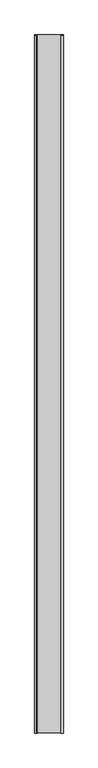
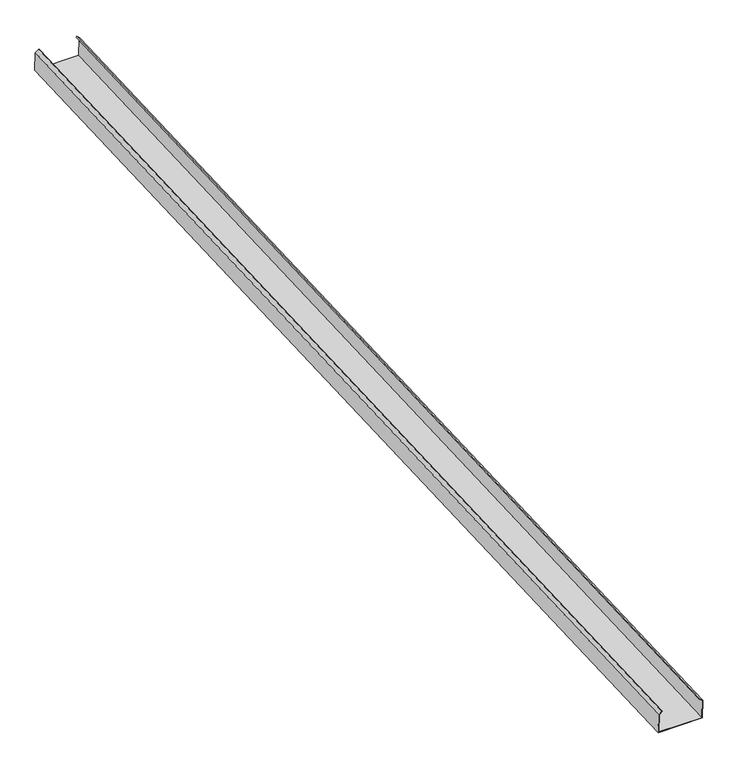
"""IFC4 building model written with IfcOpenShell, lengths in millimetres: proxy geometry, Generic Models 7:Generic Models 1:1:Generic Models 1:1 : Generic Models 7:Generic Models 1:337419:16 : Generic Models 7:Generic Models 1:1:Generic Models 1:1 : Generic Models 7:Generic Models 1:337419:306201."""

from ifc_helpers import new_model, si_unit, frame, origin, place, context, project, spatial, polyline, outline, extrude, source, transform, mapped, element, save


def generic_models_5c753bba(model_context):
    return source(origin(), model_context, "Body", "SweptSolid", [
        extrude(outline(polyline([(10.2195312, 0.0), (10.2195312, -203.2), (-78.6804688, -203.2), (-90.9255727, -188.6068534), (-88.7974056, -186.8211091), (-77.3850078, -200.421875), (7.4414063, -200.421875), (7.4414063, -2.778125), (-77.3850078, -2.778125), (-88.7974056, -16.378891), (-90.9255727, -14.5931467), (-78.6804688, 0.0), (10.2195312, 0.0)])), frame((579104.511724, -578894.7263095, 3939.1199223), z_axis=(0.0, 0.9991330730920964, 0.04163054471831409), x_axis=(0.0, 0.04163054471831409, -0.9991330730920964)), (0.0, 0.0, 1.0), 4955.6806937),
    ])


if __name__ == "__main__":
    model = new_model("IFC4")
    model_context = context("Model", 3, world=origin())
    ifc_project = project(units=[si_unit("LENGTHUNIT", "METRE", prefix="MILLI")], contexts=[model_context])
    site = spatial("IfcSite", under=ifc_project)
    building = spatial("IfcBuilding", under=site)
    placement = place(None, origin())
    generic_models_shape = generic_models_5c753bba(model_context)
    element("IfcBuildingElementProxy", 1, Name="Generic Models 7:Generic Models 1:1:Generic Models 1:1 : Generic Models 7:Generic Models 1:337419:16 : Generic Models 7:Generic Models 1:1:Generic Models 1:1 : Generic Models 7:Generic Models 1:337419:306201", ObjectType="Generic Models 7:Generic Models 1:1:Generic Models 1:1 : Generic Models 7:Generic Models 1:337419:16 : Generic Models 7:Generic Models 1:1:Generic Models 1:1 : Generic Models 7:Generic Models 1:337419:306201", at=placement, inside=building, context=model_context, shape_type="MappedRepresentation", body=[
        mapped(generic_models_shape, transform((0.0, 0.0, 0.0), x_axis=(1.0, 0.0, 0.0), y_axis=(0.0, 1.0, 0.0), z_axis=(0.0, 0.0, 1.0))),
    ])
    save(model, "model.ifc")

# Revit data of these elements
# Type "Generic Models 7:Generic Models 1:1:Generic Models 1:1 : Generic Models 7:Generic Models 1:337419:16 : Generic Models 7:Generic Models 1:1:Generic Models 1:1 : Generic Models 7:Generic Models 1:337419:306201"
#   NameOverride = "Generic Models 7:Generic Models 1:1:Generic Models 1:1 : Generic Models 7:Generic Models 1:337419:306201"
#   ObjectTypeOverride = "Generic Models 1:1 : Generic Models 7:Generic Models 1:337419"
#   Reference = "Generic Models 1"
#   Tag = "306201"
# Element 1 (IfcBuildingElementProxy, "Generic Models 7:Generic Models 1:1:Generic Models 1:1 : Generic Models 7:Generic Models 1:337419:16 : Generic Models 7:Generic Models 1:1:Generic Models 1:1 : Generic Models 7:Generic Models 1:337419:306201")
#   Materials on its faces: "'ZEE' SECTION (8.0x3.5Z - SEE STRUCT. DWGS)"
# Materials
#   "'ZEE' SECTION (8.0x3.5Z - SEE STRUCT. DWGS)": class "Unassigned", colour RGB 210 209 208, transparency 0, Keynote = "M05121300.02", Cost = 0
